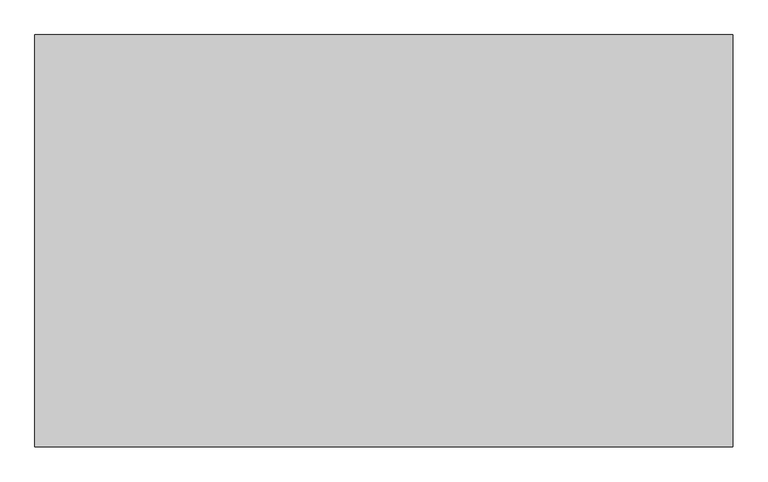
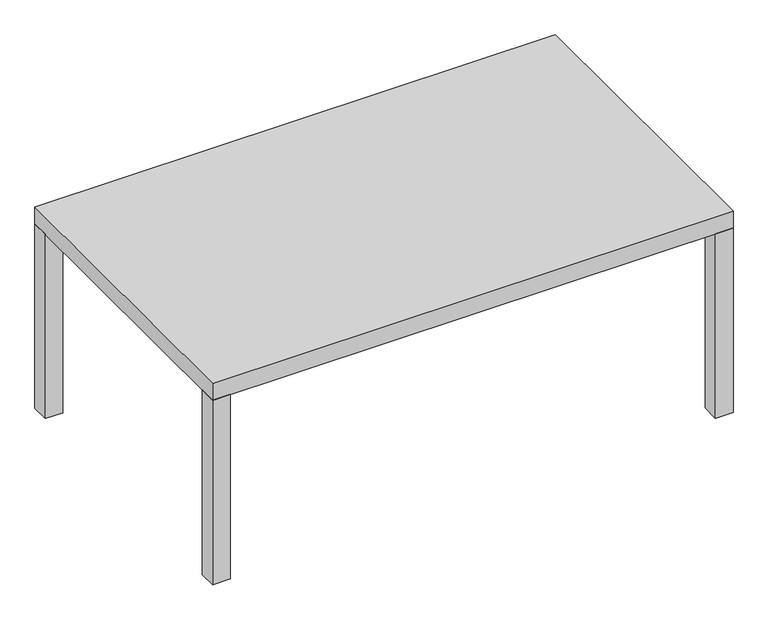
"""IFC4 building model written with IfcOpenShell, lengths in millimetres: furniture geometry, Table, Coffee-NON-COLLECTUS : -."""

from ifc_helpers import new_model, si_unit, frame, origin, origin_with_axes, place, context, project, spatial, polyline, outline, extrude, source, transform, mapped, element, save


def furniture_c2e56ca1(model_context):
    return source(origin(), model_context, "Body", "SweptSolid", [
        extrude(outline(polyline([(0.0, -622.3), (38.1, -622.3), (38.1, -660.4), (0.0, -660.4), (0.0, -622.3)])), origin_with_axes(), (0.0, 0.0, 1.0), 419.1),
        extrude(outline(polyline([(0.0, 0.0), (38.1, 0.0), (38.1, -38.1), (0.0, -38.1), (0.0, 0.0)])), origin_with_axes(), (0.0, 0.0, 1.0), 419.1),
        extrude(outline(polyline([(1117.6, -660.4), (1079.5, -660.4), (1079.5, -622.3), (1117.6, -622.3), (1117.6, -660.4)])), origin_with_axes(), (0.0, 0.0, 1.0), 419.1),
        extrude(outline(polyline([(1117.6, -38.1), (1079.5, -38.1), (1079.5, 0.0), (1117.6, 0.0), (1117.6, -38.1)])), origin_with_axes(), (0.0, 0.0, 1.0), 419.1),
        extrude(outline(polyline([(1117.6, -660.4), (0.0, -660.4), (0.0, 0.0), (1117.6, 0.0), (1117.6, -660.4)])), frame((0.0, 0.0, 419.1), z_axis=(0.0, 0.0, 1.0), x_axis=(1.0, 0.0, 0.0)), (0.0, 0.0, 1.0), 38.1),
    ])


if __name__ == "__main__":
    model = new_model("IFC4")
    model_context = context("Model", 3, world=origin())
    ifc_project = project(units=[si_unit("LENGTHUNIT", "METRE", prefix="MILLI")], contexts=[model_context])
    site = spatial("IfcSite", under=ifc_project)
    building = spatial("IfcBuilding", under=site)
    placement = place(None, origin())
    furniture_shape = furniture_c2e56ca1(model_context)
    element("IfcFurniture", 1, ObjectType="Table, Coffee-NON-COLLECTUS : -", at=placement, inside=building, context=model_context, shape_type="MappedRepresentation", body=[
        mapped(furniture_shape, transform((0.0, 0.0, 0.0), x_axis=(1.0, 0.0, 0.0), y_axis=(0.0, 1.0, 0.0), z_axis=(0.0, 0.0, 1.0))),
    ])
    save(model, "model.ifc")

# Revit data of these elements
# Type "Table, Coffee-NON-COLLECTUS : -"
#   External ID [instance default] = ""
#   Width = 1117.6 mm
#   Table Leg Size = 38.1 mm
#   Height = 457.2 mm
#   Depth = 660.4 mm
#   Material = White
#   Default Elevation = 0
# Element 1 (IfcFurniture, "Table, Coffee-NON-COLLECTUS : -")
#   Materials on its faces: "White"
# Materials
#   "White": class "Generic", colour RGB 255 255 255, transparency 0, Cost = 0
